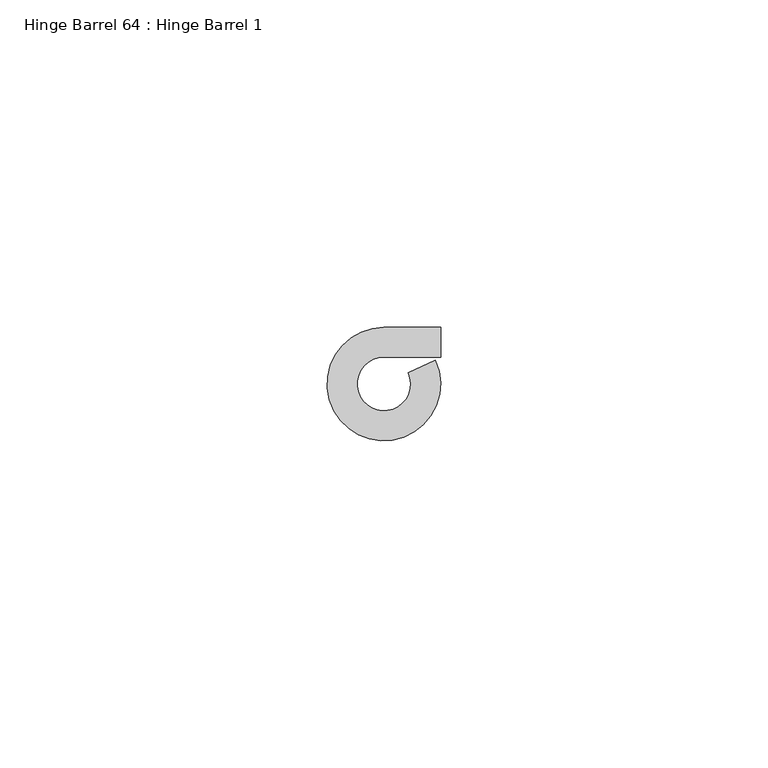
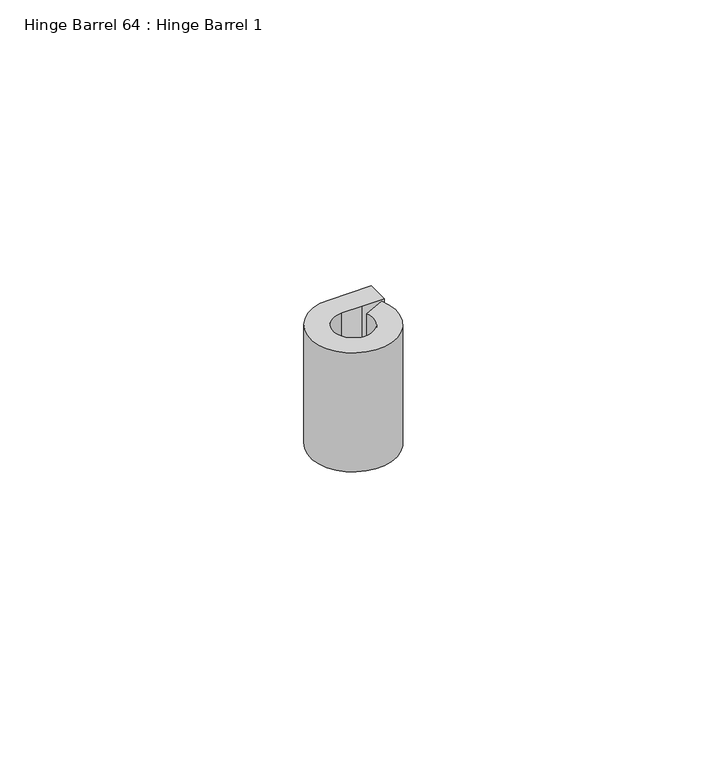
"""IFC4 building model written with IfcOpenShell, lengths in millimetres: proxy geometry, Hinge Barrel 64 : Hinge Barrel 1."""

from ifc_helpers import new_model, si_unit, point, frame, frame_2d, origin, place, context, project, spatial, polyline, circle_curve, trimmed, segment, composite_curve, outline, extrude, source, transform, mapped, element, save


def hinge_barrel_64_hinge_barrel_1_8ace309c(model_context):
    return source(origin(), model_context, "Body", "SweptSolid", [
        extrude(outline(composite_curve([segment(polyline([(587323.2214739, -536306.2758841), (587319.1320739, -536306.2758841)]), True, "CONTINUOUS"), segment(trimmed(circle_curve(frame_2d((587319.1320739, -536310.3652841)), 4.0894), [point((587319.1320739, -536306.2758841))], [point((587322.8436736, -536308.6485371))], True, "CARTESIAN"), True, "CONTINUOUS"), segment(polyline([(587322.8436736, -536308.6485371), (587326.986084, -536306.7325249)]), True, "CONTINUOUS"), segment(trimmed(circle_curve(frame_2d((587319.1320739, -536310.3652841)), 8.6534625), [point((587326.986084, -536306.7325249))], [point((587319.1320739, -536301.7118216))], False, "CARTESIAN"), True, "CONTINUOUS"), segment(polyline([(587319.1320739, -536301.7118216), (587327.7934739, -536301.7118216), (587327.7934739, -536306.2758841), (587323.2214739, -536306.2758841)]), True, "CONTINUOUS")], self_intersect=False)), frame((0.0, 0.0, 2038.35), z_axis=(0.0, 0.0, 1.0), x_axis=(1.0, 0.0, 0.0)), (0.0, 0.0, 1.0), 25.4),
    ])


if __name__ == "__main__":
    model = new_model("IFC4")
    model_context = context("Model", 3, world=origin())
    ifc_project = project(units=[si_unit("LENGTHUNIT", "METRE", prefix="MILLI")], contexts=[model_context])
    site = spatial("IfcSite", under=ifc_project)
    building = spatial("IfcBuilding", under=site)
    placement = place(None, origin())
    hinge_barrel_64_hinge_barrel_1_shape = hinge_barrel_64_hinge_barrel_1_8ace309c(model_context)
    element("IfcBuildingElementProxy", 1, Name="Hinge Barrel 64 : Hinge Barrel 1", ObjectType="Hinge Barrel 64 : Hinge Barrel 1", at=placement, inside=building, context=model_context, shape_type="MappedRepresentation", body=[
        mapped(hinge_barrel_64_hinge_barrel_1_shape, transform((0.0, 0.0, 0.0), x_axis=(1.0, 0.0, 0.0), y_axis=(0.0, 1.0, 0.0), z_axis=(0.0, 0.0, 1.0))),
    ])
    save(model, "model.ifc")

# Revit data of these elements
# Element 1 (IfcBuildingElementProxy, "Hinge Barrel 64 : Hinge Barrel 1")
#   Materials on its faces: "6\"X6\" WELD-ON STL BUTT HINGE"
# Materials
#   "6\"X6\" WELD-ON STL BUTT HINGE": class "Metal", colour RGB 189 187 185, transparency 0, Description = "Carbon steel", Cost = 0
